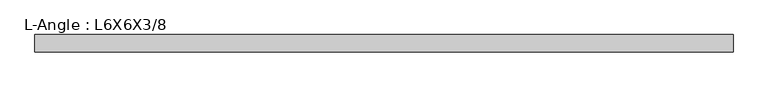
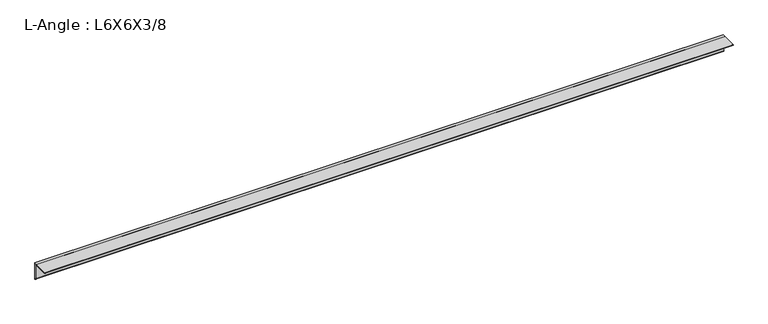
"""IFC4 building model written with IfcOpenShell, lengths in millimetres: member geometry, L-Angle : L6X6X3/8."""

import ifcopenshell
import ifcopenshell.guid

model = None  # the IFC model being written
_history = None  # IfcOwnerHistory: only IFC2X3 demands one
_inside = {}  # id of a spatial element -> (the spatial element, [elements in it])
_under = {}  # id of a project, library or spatial element -> (it, [spatial elements below it])
_declared = {}  # id of a project -> (the project, [libraries it declares])
_typed = {}  # id of a type object -> (the type object, [elements of that type])
_made_of = {}  # id of a material, layer set ... -> (it, [elements and type objects made of it])


def new_model(schema):
    """Start an empty IFC model of exactly this schema.

    Asked for "IFC4X3", IfcOpenShell would pick the latest addendum, in which some entities
    have other attributes; the version numbers below select the first issue.
    IFC2X3 requires an IfcOwnerHistory on every rooted entity: one is made here for all.
    """
    global model, _history
    if schema == "IFC4X3":
        model = ifcopenshell.file(schema_version=(4, 3, 0, 0))
    else:
        model = ifcopenshell.file(schema=schema)
    _inside.clear()
    _under.clear()
    _declared.clear()
    _typed.clear()
    _made_of.clear()
    _history = None
    if model.schema == "IFC2X3":
        org = make("IfcOrganization", Name="unknown")
        user = make(
            "IfcPersonAndOrganization",
            ThePerson=make("IfcPerson", FamilyName="unknown"),
            TheOrganization=org,
        )
        app = make(
            "IfcApplication",
            ApplicationDeveloper=org,
            Version="unknown",
            ApplicationFullName="unknown",
            ApplicationIdentifier="unknown",
        )
        _history = make(
            "IfcOwnerHistory",
            OwningUser=user,
            OwningApplication=app,
            ChangeAction="ADDED",
            CreationDate=0,
        )
    return model


def make(cls, **values):
    """One entity of the class cls with the attributes given. An attribute that is None is left unset."""
    return model.create_entity(
        cls, **{name: value for name, value in values.items() if value is not None}
    )


def rooted(cls, **values):
    """An entity with a GlobalId (a new one), such as an element, a storey or a relation."""
    return make(cls, GlobalId=ifcopenshell.guid.new(), OwnerHistory=_history, **values)


def si_unit(unit_type, name, prefix=None):
    """IfcSIUnit, for example si_unit("LENGTHUNIT", "METRE", prefix="MILLI")."""
    return make("IfcSIUnit", UnitType=unit_type, Prefix=prefix, Name=name)


def assignment(units):
    """IfcUnitAssignment: the units of a project."""
    return None if units is None else make("IfcUnitAssignment", Units=units)


def point(xyz):
    """IfcCartesianPoint."""
    return None if xyz is None else make("IfcCartesianPoint", Coordinates=xyz)


def direction(xyz):
    """IfcDirection."""
    return None if xyz is None else make("IfcDirection", DirectionRatios=xyz)


def frame(location, z_axis=None, x_axis=None):
    """IfcAxis2Placement3D, a coordinate frame: its origin and axes. An axis left out is left unset."""
    return make(
        "IfcAxis2Placement3D",
        Location=point(location),
        Axis=direction(z_axis),
        RefDirection=direction(x_axis),
    )


def frame_2d(location, x_axis=None):
    """IfcAxis2Placement2D, a coordinate frame in the plane: its origin and x axis."""
    return make(
        "IfcAxis2Placement2D", Location=point(location), RefDirection=direction(x_axis)
    )


def origin():
    """The frame at (0, 0, 0) with its axes left unset."""
    return frame((0.0, 0.0, 0.0))


def place(relative_to, where):
    """IfcLocalPlacement: puts the frame where relative to a parent placement (None: the world)."""
    return make(
        "IfcLocalPlacement", PlacementRelTo=relative_to, RelativePlacement=where
    )


def context(
    kind, dimensions, precision=None, world=None, true_north=None, identifier=None
):
    """IfcGeometricRepresentationContext, for example the 3D "Model" context."""
    return make(
        "IfcGeometricRepresentationContext",
        ContextIdentifier=identifier,
        ContextType=kind,
        CoordinateSpaceDimension=dimensions,
        Precision=precision,
        WorldCoordinateSystem=world,
        TrueNorth=true_north,
    )


def project(units=None, contexts=None):
    """IfcProject with its units and contexts."""
    return rooted(
        "IfcProject",
        Name="project",
        RepresentationContexts=contexts,
        UnitsInContext=assignment(units),
    )


def spatial(cls, under=None, at=None, **own):
    """A site, building, storey or space (cls), placed at a placement, below another one or the project."""
    s = rooted(cls, ObjectPlacement=at, **own)
    if under is not None:
        _under.setdefault(under.id(), (under, []))[1].append(s)
    return s


def polyline(points):
    """IfcPolyline through the points."""
    return make("IfcPolyline", Points=[point(p) for p in points])


def circle_curve(where, radius):
    """IfcCircle in the frame where."""
    return make("IfcCircle", Position=where, Radius=radius)


def trimmed(basis, trim1, trim2, sense, master):
    """IfcTrimmedCurve: the piece of a basis curve between two trims."""
    return make(
        "IfcTrimmedCurve",
        BasisCurve=basis,
        Trim1=trim1,
        Trim2=trim2,
        SenseAgreement=sense,
        MasterRepresentation=master,
    )


def segment(curve, same_sense, transition):
    """IfcCompositeCurveSegment."""
    return make(
        "IfcCompositeCurveSegment",
        Transition=transition,
        SameSense=same_sense,
        ParentCurve=curve,
    )


def composite_curve(segments, self_intersect=None):
    """IfcCompositeCurve: segments joined end to end."""
    return make("IfcCompositeCurve", Segments=segments, SelfIntersect=self_intersect)


def outline(outer, holes=None, kind="AREA"):
    """IfcArbitraryClosedProfileDef: a profile drawn as a closed curve; with holes, ...WithVoids."""
    if holes is None:
        return make("IfcArbitraryClosedProfileDef", ProfileType=kind, OuterCurve=outer)
    return make(
        "IfcArbitraryProfileDefWithVoids",
        ProfileType=kind,
        OuterCurve=outer,
        InnerCurves=holes,
    )


def extrude(swept, where, along, depth):
    """IfcExtrudedAreaSolid: the profile swept, set in the frame where, extruded along a direction by depth."""
    return make(
        "IfcExtrudedAreaSolid",
        SweptArea=swept,
        Position=where,
        ExtrudedDirection=direction(along),
        Depth=depth,
    )


def shape(context_of_items, identifier, shape_type, items):
    """IfcShapeRepresentation: the items that make up one representation, for example the "Body"."""
    return make(
        "IfcShapeRepresentation",
        ContextOfItems=context_of_items,
        RepresentationIdentifier=identifier,
        RepresentationType=shape_type,
        Items=items,
    )


def source(mapping_origin, context_of_items, identifier, shape_type, items):
    """IfcRepresentationMap: a shape defined once, which mapped items show again and again."""
    return make(
        "IfcRepresentationMap",
        MappingOrigin=mapping_origin,
        MappedRepresentation=shape(context_of_items, identifier, shape_type, items),
    )


def transform(
    local_origin,
    x_axis=None,
    y_axis=None,
    z_axis=None,
    scale=None,
    scale2=None,
    scale3=None,
    uniform=True,
):
    """IfcCartesianTransformationOperator3D, or its non-uniform kind. x_axis, y_axis, z_axis: its Axis1, 2, 3."""
    if uniform:
        return make(
            "IfcCartesianTransformationOperator3D",
            Axis1=direction(x_axis),
            Axis2=direction(y_axis),
            LocalOrigin=point(local_origin),
            Scale=scale,
            Axis3=direction(z_axis),
        )
    return make(
        "IfcCartesianTransformationOperator3DnonUniform",
        Axis1=direction(x_axis),
        Axis2=direction(y_axis),
        LocalOrigin=point(local_origin),
        Scale=scale,
        Axis3=direction(z_axis),
        Scale2=scale2,
        Scale3=scale3,
    )


def mapped(mapping_source, mapping_target):
    """IfcMappedItem: shows the shape of a source again, moved by a transform."""
    return make(
        "IfcMappedItem", MappingSource=mapping_source, MappingTarget=mapping_target
    )


def made_of(thing, what):
    """Note that an element or type object is made of a material, layer set ...; save() writes the relation."""
    if what is not None:
        _made_of.setdefault(what.id(), (what, []))[1].append(thing)
    return thing


def element(
    cls,
    number,
    at=None,
    inside=None,
    cuts=None,
    type_object=None,
    material=None,
    context=None,
    identifier="Body",
    shape_type=None,
    held_by="IfcProductDefinitionShape",
    body=None,
    shapes=None,
    **own,
):
    """One element of the class cls, such as IfcWall. Its Tag is "e" and its number.

    at: its placement. inside: the storey or other place that contains it. cuts: it is an
    opening in that element (IfcRelVoidsElement). A single representation is given by context,
    identifier, shape_type and body (its items); several are given by shapes. held_by: the class
    of the entity that holds the representations. save() writes the other relations.
    """
    e = rooted(cls, Tag="e%d" % number, ObjectPlacement=at, **own)
    if body is not None:
        shapes = [shape(context, identifier, shape_type, body)]
    if shapes is not None:
        e.Representation = make(held_by, Representations=shapes)
    if inside is not None:
        _inside.setdefault(inside.id(), (inside, []))[1].append(e)
    if cuts is not None:
        rooted(
            "IfcRelVoidsElement", RelatingBuildingElement=cuts, RelatedOpeningElement=e
        )
    if type_object is not None:
        _typed.setdefault(type_object.id(), (type_object, []))[1].append(e)
    return made_of(e, material)


def aggregate(whole, parts):
    """IfcRelAggregates: a whole, such as a stair, and the parts it consists of."""
    return rooted("IfcRelAggregates", RelatingObject=whole, RelatedObjects=parts)


def save(model, path):
    """Write the relations noted so far, then the file.

    IfcRelAggregates (storeys below a building ...), IfcRelContainedInSpatialStructure (elements
    in a storey), IfcRelDefinesByType, IfcRelAssociatesMaterial and IfcRelDeclares: one each for
    every whole, place, type object, material and project.
    """
    for whole, parts in _under.values():
        aggregate(whole, parts)
    for where, things in _inside.values():
        rooted(
            "IfcRelContainedInSpatialStructure",
            RelatedElements=things,
            RelatingStructure=where,
        )
    for kind, things in _typed.values():
        rooted("IfcRelDefinesByType", RelatedObjects=things, RelatingType=kind)
    for what, things in _made_of.values():
        rooted("IfcRelAssociatesMaterial", RelatedObjects=things, RelatingMaterial=what)
    for by, libraries in _declared.values():
        rooted("IfcRelDeclares", RelatingContext=by, RelatedDefinitions=libraries)
    model.write(path)


def l_angle_l6x6x3_8_2b984bf3(model_context):
    return source(origin(), model_context, "Body", "SweptSolid", [
        extrude(outline(composite_curve([segment(polyline([(41.148, 41.148), (41.148, -111.252)]), True, "CONTINUOUS"), segment(trimmed(circle_curve(frame_2d((41.148, -101.727)), 9.525), [point((41.148, -111.252))], [point((31.623, -101.727))], False, "CARTESIAN"), True, "CONTINUOUS"), segment(polyline([(31.623, -101.727), (31.623, 22.098)]), True, "CONTINUOUS"), segment(trimmed(circle_curve(frame_2d((22.098, 22.098)), 9.525), [point((31.623, 22.098))], [point((22.098, 31.623))], True, "CARTESIAN"), True, "CONTINUOUS"), segment(polyline([(22.098, 31.623), (-101.727, 31.623)]), True, "CONTINUOUS"), segment(trimmed(circle_curve(frame_2d((-101.727, 41.148)), 9.525), [point((-101.727, 31.623))], [point((-111.252, 41.148))], False, "CARTESIAN"), True, "CONTINUOUS"), segment(polyline([(-111.252, 41.148), (41.148, 41.148)]), True, "CONTINUOUS")], self_intersect=False)), frame((-3088.1296112, 0.0, 0.0), z_axis=(1.0, 0.0, 0.0), x_axis=(0.0, 1.0, 0.0)), (0.0, 0.0, 1.0), 6142.746295),
    ])


if __name__ == "__main__":
    model = new_model("IFC4")
    model_context = context("Model", 3, world=origin())
    ifc_project = project(units=[si_unit("LENGTHUNIT", "METRE", prefix="MILLI")], contexts=[model_context])
    site = spatial("IfcSite", under=ifc_project)
    building = spatial("IfcBuilding", under=site)
    placement = place(None, origin())
    l_angle_l6x6x3_8_shape = l_angle_l6x6x3_8_2b984bf3(model_context)
    element("IfcMember", 1, ObjectType="L-Angle : L6X6X3/8", at=placement, inside=building, context=model_context, shape_type="MappedRepresentation", body=[
        mapped(l_angle_l6x6x3_8_shape, transform((0.0, 0.0, 0.0), x_axis=(1.0, 0.0, 0.0), y_axis=(0.0, 1.0, 0.0), z_axis=(0.0, 0.0, 1.0))),
    ])
    save(model, "model.ifc")

# Revit data of these elements
# Type "L-Angle : L6X6X3/8"
#   Assembly Code = "B10"
#   k = 0' - 0 7/8"
#   W = 14.9
#   Length [instance default] = 5' - 0"
#   b = 0' - 6"
#   d = 0' - 6"
#   t = 0' - 0 3/8"
#   x = 0' - 1.62"
#   y = 0' - 1.62"
#   A = 0.0304167 SF
#   Structural Material [instance default] = Steel ASTM A36
# Element 1 (IfcMember, "L-Angle : L6X6X3/8")
#   Materials on its faces: "Steel ASTM A36"
# Materials
#   "Steel ASTM A36": class "Metal", colour RGB 199 199 199, transparency 0, Description = "Structural steel, ASTM A36 Grade B, mill finish", Cost = 0
